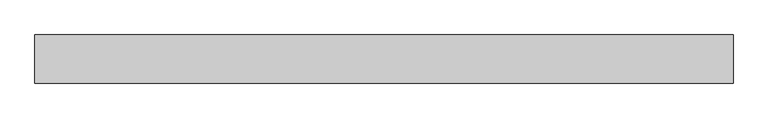
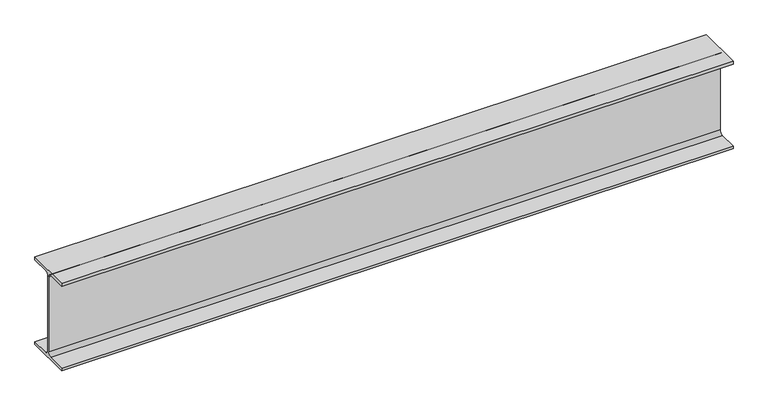
"""IFC4 building model written with IfcOpenShell, lengths in millimetres: beam geometry, 0912_Steel Framing_H-KSD3502 : H_SB_ASB_H-350x175x7x11."""

from ifc_helpers import new_model, si_unit, point, frame, frame_2d, origin, place, context, project, spatial, polyline, circle_curve, trimmed, segment, composite_curve, outline, extrude, source, transform, mapped, element, save


def beam_0f635493(model_context):
    return source(origin(), model_context, "Body", "SweptSolid", [
        extrude(outline(composite_curve([segment(polyline([(87.5, -164.0), (87.5, -175.0), (-87.5, -175.0), (-87.5, -164.0), (-17.5, -164.0)]), True, "CONTINUOUS"), segment(trimmed(circle_curve(frame_2d((-17.5, -150.0)), 14.0), [point((-17.5, -164.0))], [point((-3.5, -150.0))], True, "CARTESIAN"), True, "CONTINUOUS"), segment(polyline([(-3.5, -150.0), (-3.5, 150.0)]), True, "CONTINUOUS"), segment(trimmed(circle_curve(frame_2d((-17.5, 150.0)), 14.0), [point((-3.5, 150.0))], [point((-17.5, 164.0))], True, "CARTESIAN"), True, "CONTINUOUS"), segment(polyline([(-17.5, 164.0), (-87.5, 164.0), (-87.5, 175.0), (87.5, 175.0), (87.5, 164.0), (17.5, 164.0)]), True, "CONTINUOUS"), segment(trimmed(circle_curve(frame_2d((17.5, 150.0)), 14.0), [point((17.5, 164.0))], [point((3.5, 150.0))], True, "CARTESIAN"), True, "CONTINUOUS"), segment(polyline([(3.5, 150.0), (3.5, -150.0)]), True, "CONTINUOUS"), segment(trimmed(circle_curve(frame_2d((17.5, -150.0)), 14.0), [point((3.5, -150.0))], [point((17.5, -164.0))], True, "CARTESIAN"), True, "CONTINUOUS"), segment(polyline([(17.5, -164.0), (87.5, -164.0)]), True, "CONTINUOUS")], self_intersect=False)), frame((-1295.7739051, 0.0, 0.0), z_axis=(1.0, 0.0, 0.0), x_axis=(0.0, 1.0, 0.0)), (0.0, 0.0, 1.0), 2540.0189947),
    ])


if __name__ == "__main__":
    model = new_model("IFC4")
    model_context = context("Model", 3, world=origin())
    ifc_project = project(units=[si_unit("LENGTHUNIT", "METRE", prefix="MILLI")], contexts=[model_context])
    site = spatial("IfcSite", under=ifc_project)
    building = spatial("IfcBuilding", under=site)
    placement = place(None, origin())
    beam_shape = beam_0f635493(model_context)
    element("IfcBeam", 1, ObjectType="0912_Steel Framing_H-KSD3502 : H_SB_ASB_H-350x175x7x11", at=placement, inside=building, context=model_context, shape_type="MappedRepresentation", body=[
        mapped(beam_shape, transform((0.0, 0.0, 0.0), x_axis=(1.0, 0.0, 0.0), y_axis=(0.0, 1.0, 0.0), z_axis=(0.0, 0.0, 1.0))),
    ])
    save(model, "model.ifc")

# Revit data of these elements
# Type "0912_Steel Framing_H-KSD3502 : H_SB_ASB_H-350x175x7x11"
#   H_WM Code_1 = "S01AA002-00001 | Main Steel Structure Fabrication Work | Shelter/Building | Medium Steel - Standard (90KG/M>Weight≥30KG/M) | Material: (   )"
#   H_WM Code_2 = "S03AA028-00001 | Main Steel Structure Erection Work | Shelter/Building | Medium Steel (90KG/M>Weight≥30KG/M) | Material: (   )"
#   H_WM Code_3 = "S01AA010-00001 | Main Steel Structure Fabrication Work | Shelter/Building | Steel Painting/Coating | for Non-Fireproofed Steel Surface, Surface Preparation, Primer, Second & Final Coat | Material: (   )"
#   H_Q'ty Cal Type Tag = "SB-Q2"
#   Width = 17.5 cm
#   Web Thickness = 0.7 cm
#   Web Fillet = 1.4 cm
#   Warping Constant = 282000.0 cm⁶
#   W = 0
#   Torsional Moment of Inertia = 19.4042 cm⁴
#   Section Area = 63.14 cm²
#   Plastic Modulus weak axis = 174.0 cm³
#   Plastic Modulus strong axis = 868.0 cm³
#   Perimeter = 1.36 m²/m
#   Nominal Weight = 49.60 kgf/m
#   Moment of Inertia weak axis = 984.00 cm⁴
#   Moment of Inertia strong axis = 13600.00 cm⁴
#   Height = 35.0 cm
#   Flange Thickness = 1.1 cm
#   Elastic Modulus weak axis = 112.0 cm³
#   Elastic Modulus strong axis = 775.0 cm³
#   Centroid Vertical = 17.5 cm
#   Centroid Horizontal = 8.75 cm
#   Ix = 136000000
#   Length [instance default] = 1.5240 m
#   Zx = 868000
#   b = 0.1750 m
#   h = 0.3500 m
#   r = 0.0140 m
#   s = 0.0070 m
#   t = 0.0110 m
#   A = 0.006314 m²
#   Structural Material [instance default] = Steel, 45-345
#   Assembly Code = ""
# Element 1 (IfcBeam, "0912_Steel Framing_H-KSD3502 : H_SB_ASB_H-350x175x7x11")
#   Structural Material = none
# Materials
#   "Steel, 45-345": class "Metal", colour RGB 189 187 185, transparency 0, Description = "Steel 345 MPa", Cost = 0
